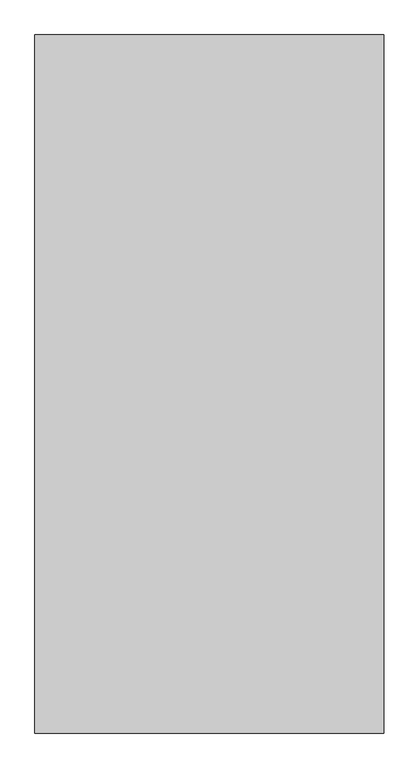
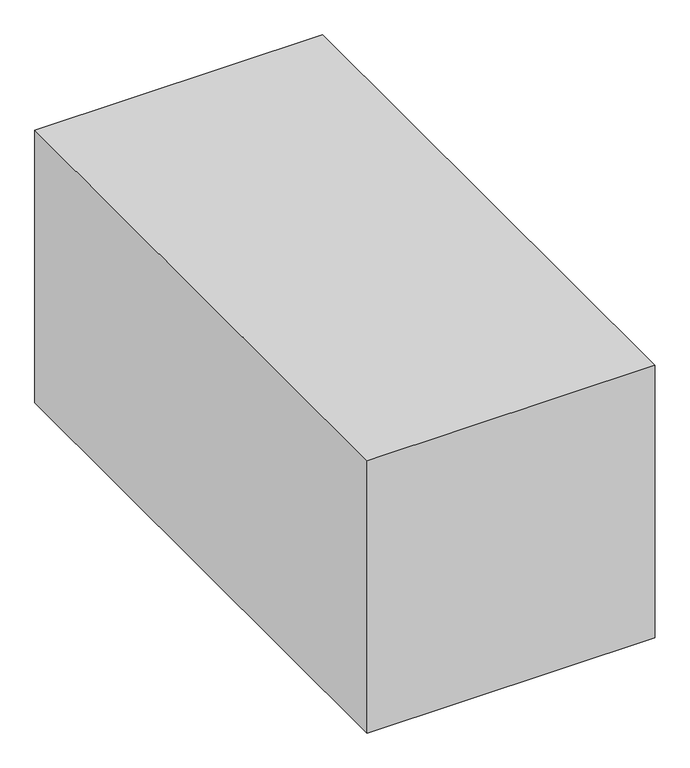
"""IFC4 building model written with IfcOpenShell, lengths in millimetres: proxy geometry, Space Planning Box_hec : Space Planning Box_hec."""

import ifcopenshell
import ifcopenshell.guid

model = None  # the IFC model being written
_history = None  # IfcOwnerHistory: only IFC2X3 demands one
_inside = {}  # id of a spatial element -> (the spatial element, [elements in it])
_under = {}  # id of a project, library or spatial element -> (it, [spatial elements below it])
_declared = {}  # id of a project -> (the project, [libraries it declares])
_typed = {}  # id of a type object -> (the type object, [elements of that type])
_made_of = {}  # id of a material, layer set ... -> (it, [elements and type objects made of it])


def new_model(schema):
    """Start an empty IFC model of exactly this schema.

    Asked for "IFC4X3", IfcOpenShell would pick the latest addendum, in which some entities
    have other attributes; the version numbers below select the first issue.
    IFC2X3 requires an IfcOwnerHistory on every rooted entity: one is made here for all.
    """
    global model, _history
    if schema == "IFC4X3":
        model = ifcopenshell.file(schema_version=(4, 3, 0, 0))
    else:
        model = ifcopenshell.file(schema=schema)
    _inside.clear()
    _under.clear()
    _declared.clear()
    _typed.clear()
    _made_of.clear()
    _history = None
    if model.schema == "IFC2X3":
        org = make("IfcOrganization", Name="unknown")
        user = make(
            "IfcPersonAndOrganization",
            ThePerson=make("IfcPerson", FamilyName="unknown"),
            TheOrganization=org,
        )
        app = make(
            "IfcApplication",
            ApplicationDeveloper=org,
            Version="unknown",
            ApplicationFullName="unknown",
            ApplicationIdentifier="unknown",
        )
        _history = make(
            "IfcOwnerHistory",
            OwningUser=user,
            OwningApplication=app,
            ChangeAction="ADDED",
            CreationDate=0,
        )
    return model


def make(cls, **values):
    """One entity of the class cls with the attributes given. An attribute that is None is left unset."""
    return model.create_entity(
        cls, **{name: value for name, value in values.items() if value is not None}
    )


def rooted(cls, **values):
    """An entity with a GlobalId (a new one), such as an element, a storey or a relation."""
    return make(cls, GlobalId=ifcopenshell.guid.new(), OwnerHistory=_history, **values)


def si_unit(unit_type, name, prefix=None):
    """IfcSIUnit, for example si_unit("LENGTHUNIT", "METRE", prefix="MILLI")."""
    return make("IfcSIUnit", UnitType=unit_type, Prefix=prefix, Name=name)


def assignment(units):
    """IfcUnitAssignment: the units of a project."""
    return None if units is None else make("IfcUnitAssignment", Units=units)


def point(xyz):
    """IfcCartesianPoint."""
    return None if xyz is None else make("IfcCartesianPoint", Coordinates=xyz)


def direction(xyz):
    """IfcDirection."""
    return None if xyz is None else make("IfcDirection", DirectionRatios=xyz)


def frame(location, z_axis=None, x_axis=None):
    """IfcAxis2Placement3D, a coordinate frame: its origin and axes. An axis left out is left unset."""
    return make(
        "IfcAxis2Placement3D",
        Location=point(location),
        Axis=direction(z_axis),
        RefDirection=direction(x_axis),
    )


def origin():
    """The frame at (0, 0, 0) with its axes left unset."""
    return frame((0.0, 0.0, 0.0))


def origin_with_axes():
    """The frame at (0, 0, 0) with the z axis (0, 0, 1) and the x axis (1, 0, 0) written out."""
    return frame((0.0, 0.0, 0.0), z_axis=(0.0, 0.0, 1.0), x_axis=(1.0, 0.0, 0.0))


def place(relative_to, where):
    """IfcLocalPlacement: puts the frame where relative to a parent placement (None: the world)."""
    return make(
        "IfcLocalPlacement", PlacementRelTo=relative_to, RelativePlacement=where
    )


def context(
    kind, dimensions, precision=None, world=None, true_north=None, identifier=None
):
    """IfcGeometricRepresentationContext, for example the 3D "Model" context."""
    return make(
        "IfcGeometricRepresentationContext",
        ContextIdentifier=identifier,
        ContextType=kind,
        CoordinateSpaceDimension=dimensions,
        Precision=precision,
        WorldCoordinateSystem=world,
        TrueNorth=true_north,
    )


def project(units=None, contexts=None):
    """IfcProject with its units and contexts."""
    return rooted(
        "IfcProject",
        Name="project",
        RepresentationContexts=contexts,
        UnitsInContext=assignment(units),
    )


def spatial(cls, under=None, at=None, **own):
    """A site, building, storey or space (cls), placed at a placement, below another one or the project."""
    s = rooted(cls, ObjectPlacement=at, **own)
    if under is not None:
        _under.setdefault(under.id(), (under, []))[1].append(s)
    return s


def polyline(points):
    """IfcPolyline through the points."""
    return make("IfcPolyline", Points=[point(p) for p in points])


def outline(outer, holes=None, kind="AREA"):
    """IfcArbitraryClosedProfileDef: a profile drawn as a closed curve; with holes, ...WithVoids."""
    if holes is None:
        return make("IfcArbitraryClosedProfileDef", ProfileType=kind, OuterCurve=outer)
    return make(
        "IfcArbitraryProfileDefWithVoids",
        ProfileType=kind,
        OuterCurve=outer,
        InnerCurves=holes,
    )


def extrude(swept, where, along, depth):
    """IfcExtrudedAreaSolid: the profile swept, set in the frame where, extruded along a direction by depth."""
    return make(
        "IfcExtrudedAreaSolid",
        SweptArea=swept,
        Position=where,
        ExtrudedDirection=direction(along),
        Depth=depth,
    )


def shape(context_of_items, identifier, shape_type, items):
    """IfcShapeRepresentation: the items that make up one representation, for example the "Body"."""
    return make(
        "IfcShapeRepresentation",
        ContextOfItems=context_of_items,
        RepresentationIdentifier=identifier,
        RepresentationType=shape_type,
        Items=items,
    )


def source(mapping_origin, context_of_items, identifier, shape_type, items):
    """IfcRepresentationMap: a shape defined once, which mapped items show again and again."""
    return make(
        "IfcRepresentationMap",
        MappingOrigin=mapping_origin,
        MappedRepresentation=shape(context_of_items, identifier, shape_type, items),
    )


def transform(
    local_origin,
    x_axis=None,
    y_axis=None,
    z_axis=None,
    scale=None,
    scale2=None,
    scale3=None,
    uniform=True,
):
    """IfcCartesianTransformationOperator3D, or its non-uniform kind. x_axis, y_axis, z_axis: its Axis1, 2, 3."""
    if uniform:
        return make(
            "IfcCartesianTransformationOperator3D",
            Axis1=direction(x_axis),
            Axis2=direction(y_axis),
            LocalOrigin=point(local_origin),
            Scale=scale,
            Axis3=direction(z_axis),
        )
    return make(
        "IfcCartesianTransformationOperator3DnonUniform",
        Axis1=direction(x_axis),
        Axis2=direction(y_axis),
        LocalOrigin=point(local_origin),
        Scale=scale,
        Axis3=direction(z_axis),
        Scale2=scale2,
        Scale3=scale3,
    )


def mapped(mapping_source, mapping_target):
    """IfcMappedItem: shows the shape of a source again, moved by a transform."""
    return make(
        "IfcMappedItem", MappingSource=mapping_source, MappingTarget=mapping_target
    )


def made_of(thing, what):
    """Note that an element or type object is made of a material, layer set ...; save() writes the relation."""
    if what is not None:
        _made_of.setdefault(what.id(), (what, []))[1].append(thing)
    return thing


def element(
    cls,
    number,
    at=None,
    inside=None,
    cuts=None,
    type_object=None,
    material=None,
    context=None,
    identifier="Body",
    shape_type=None,
    held_by="IfcProductDefinitionShape",
    body=None,
    shapes=None,
    **own,
):
    """One element of the class cls, such as IfcWall. Its Tag is "e" and its number.

    at: its placement. inside: the storey or other place that contains it. cuts: it is an
    opening in that element (IfcRelVoidsElement). A single representation is given by context,
    identifier, shape_type and body (its items); several are given by shapes. held_by: the class
    of the entity that holds the representations. save() writes the other relations.
    """
    e = rooted(cls, Tag="e%d" % number, ObjectPlacement=at, **own)
    if body is not None:
        shapes = [shape(context, identifier, shape_type, body)]
    if shapes is not None:
        e.Representation = make(held_by, Representations=shapes)
    if inside is not None:
        _inside.setdefault(inside.id(), (inside, []))[1].append(e)
    if cuts is not None:
        rooted(
            "IfcRelVoidsElement", RelatingBuildingElement=cuts, RelatedOpeningElement=e
        )
    if type_object is not None:
        _typed.setdefault(type_object.id(), (type_object, []))[1].append(e)
    return made_of(e, material)


def aggregate(whole, parts):
    """IfcRelAggregates: a whole, such as a stair, and the parts it consists of."""
    return rooted("IfcRelAggregates", RelatingObject=whole, RelatedObjects=parts)


def save(model, path):
    """Write the relations noted so far, then the file.

    IfcRelAggregates (storeys below a building ...), IfcRelContainedInSpatialStructure (elements
    in a storey), IfcRelDefinesByType, IfcRelAssociatesMaterial and IfcRelDeclares: one each for
    every whole, place, type object, material and project.
    """
    for whole, parts in _under.values():
        aggregate(whole, parts)
    for where, things in _inside.values():
        rooted(
            "IfcRelContainedInSpatialStructure",
            RelatedElements=things,
            RelatingStructure=where,
        )
    for kind, things in _typed.values():
        rooted("IfcRelDefinesByType", RelatedObjects=things, RelatingType=kind)
    for what, things in _made_of.values():
        rooted("IfcRelAssociatesMaterial", RelatedObjects=things, RelatingMaterial=what)
    for by, libraries in _declared.values():
        rooted("IfcRelDeclares", RelatingContext=by, RelatedDefinitions=libraries)
    model.write(path)


def generic_models_43059f4e(model_context):
    return source(origin(), model_context, "Body", "SweptSolid", [
        extrude(outline(polyline([(3000.0, 6000.0), (3000.0, -6000.0), (-3000.0, -6000.0), (-3000.0, 6000.0), (3000.0, 6000.0)])), origin_with_axes(), (0.0, 0.0, 1.0), 6000.0),
    ])


if __name__ == "__main__":
    model = new_model("IFC4")
    model_context = context("Model", 3, world=origin())
    ifc_project = project(units=[si_unit("LENGTHUNIT", "METRE", prefix="MILLI")], contexts=[model_context])
    site = spatial("IfcSite", under=ifc_project)
    building = spatial("IfcBuilding", under=site)
    placement = place(None, origin())
    generic_models_shape = generic_models_43059f4e(model_context)
    element("IfcBuildingElementProxy", 1, Name="Space Planning Box_hec : Space Planning Box_hec", ObjectType="Space Planning Box_hec : Space Planning Box_hec", at=placement, inside=building, context=model_context, shape_type="MappedRepresentation", body=[
        mapped(generic_models_shape, transform((0.0, 0.0, 0.0), x_axis=(1.0, 0.0, 0.0), y_axis=(0.0, 1.0, 0.0), z_axis=(0.0, 0.0, 1.0))),
    ])
    save(model, "model.ifc")

# Revit data of these elements
# Type "Space Planning Box_hec : Space Planning Box_hec"
#   Type Comments = "..."
#   Room Name [instance default] = "?"
#   Interior Finish [instance default] = ""
#   Exterior Finish [instance default] = ""
#   Department [instance default] = ""
#   Assembly Code = "..."
#   Width [instance default] = 1524 mm
#   Program Area [instance default] = 0.00 m²
#   Length [instance default] = 1524 mm
#   Height [instance default] = 1524 mm
#   Area [instance default] = 2.32258 m²
#   Fill Color [instance default] = Cyan
#   Default Elevation = 0
# Element 1 (IfcBuildingElementProxy, "Space Planning Box_hec : Space Planning Box_hec")
#   Room Name = "Toilet (M)"
#   Interior Finish = "IF5"
#   Exterior Finish = "EF1"
#   Department = "AR"
#   Width = 6000 mm
#   Program Area = 72.00 m²
#   Length = 12000 mm
#   Height = 6000 mm
#   Area = 72.00 m²
#   Fill Color = Lavender
#   Materials on its faces: "Lavender"
# Materials
#   "Cyan": class "Generic", colour RGB 0 255 255, transparency 0.2, Cost = 0
#   "Lavender": class "Generic", colour RGB 186 85 211, transparency 0.2, Cost = 0
